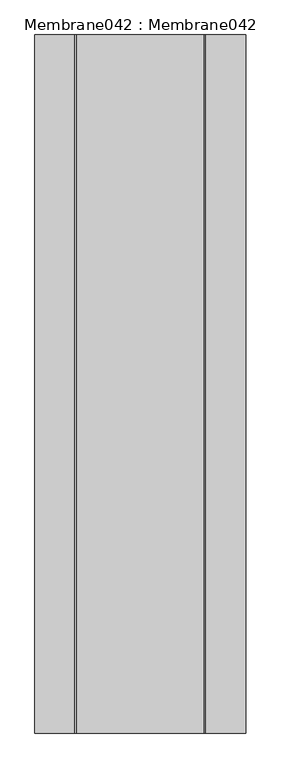
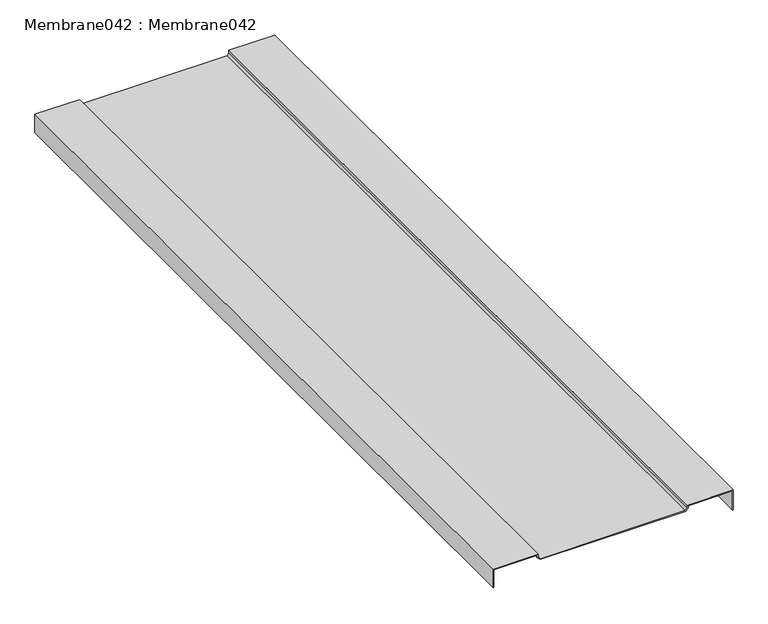
"""IFC4 building model written with IfcOpenShell, lengths in millimetres: proxy geometry, Membrane042 : Membrane042."""

from ifc_helpers import new_model, si_unit, frame, origin, place, context, project, spatial, polyline, outline, extrude, source, transform, mapped, element, save


def membrane042_membrane042_7156602d(model_context):
    return source(origin(), model_context, "Body", "SweptSolid", [
        extrude(outline(polyline([(40067.8433955, -9290.6521637), (40120.3473017, -9290.6521637), (40120.3473017, -9406.2119141), (40112.7345471, -9406.2119141), (40107.5625, -9410.821371), (40107.5625, -9776.0706055), (40113.484858, -9782.1787109), (40120.9432079, -9782.1787109), (40120.9432079, -9895.1605691), (40071.8338329, -9895.1605691), (40071.8338329, -9893.1605691), (40118.9432079, -9893.1605691), (40118.9432079, -9784.1787109), (40112.6382852, -9784.1787109), (40105.5625, -9776.8810025), (40105.5625, -9409.9248047), (40111.9726562, -9404.2119141), (40118.3473017, -9404.2119141), (40118.3473017, -9292.6521637), (40067.8433955, -9292.6521637), (40067.8433955, -9290.6521637)])), frame((0.0, 7182.1531721, 0.0), z_axis=(0.0, 1.0, 0.0), x_axis=(0.0, 0.0, 1.0)), (0.0, 0.0, 1.0), 2000.0),
    ])


if __name__ == "__main__":
    model = new_model("IFC4")
    model_context = context("Model", 3, world=origin())
    ifc_project = project(units=[si_unit("LENGTHUNIT", "METRE", prefix="MILLI")], contexts=[model_context])
    site = spatial("IfcSite", under=ifc_project)
    building = spatial("IfcBuilding", under=site)
    placement = place(None, origin())
    membrane042_membrane042_shape = membrane042_membrane042_7156602d(model_context)
    element("IfcBuildingElementProxy", 1, Name="Membrane042 : Membrane042", ObjectType="Membrane042 : Membrane042", at=placement, inside=building, context=model_context, shape_type="MappedRepresentation", body=[
        mapped(membrane042_membrane042_shape, transform((0.0, 0.0, 0.0), x_axis=(1.0, 0.0, 0.0), y_axis=(0.0, 1.0, 0.0), z_axis=(0.0, 0.0, 1.0))),
    ])
    save(model, "model.ifc")

# Revit data of these elements
# Type "Membrane042 : Membrane042"
#   NameOverride = "Membrane042"
# Element 1 (IfcBuildingElementProxy, "Membrane042 : Membrane042")
#   Materials on its faces: "WESTCOAT ALX UNDER TILE WATERPROOFING SYSTEM (FOLLOW MANUFACTURER'S INSTALLATION REQUIREMENTS)"
# Materials
#   "WESTCOAT ALX UNDER TILE WATERPROOFING SYSTEM (FOLLOW MANUFACTURER'S INSTALLATION REQUIREMENTS)": class "Unassigned", colour RGB 179 255 168, transparency 0, Cost = 0
